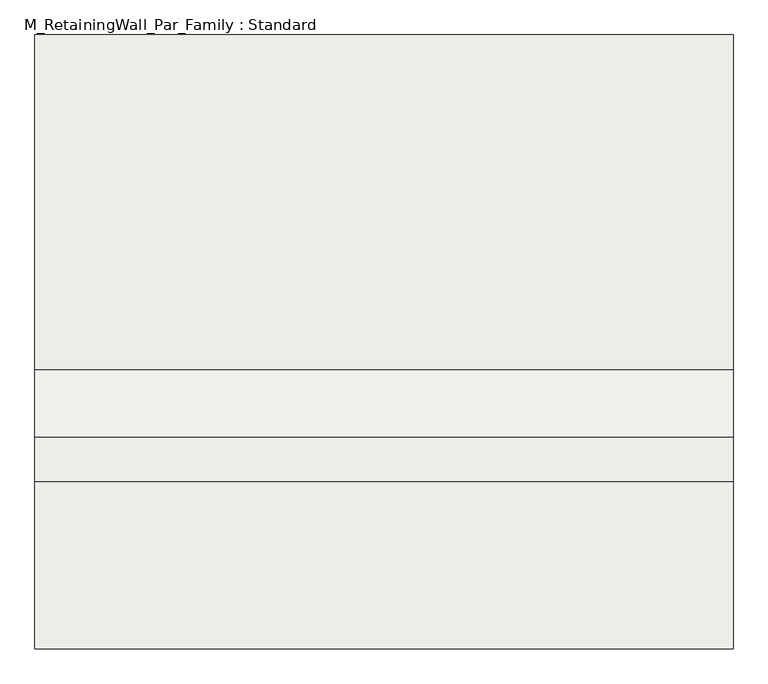
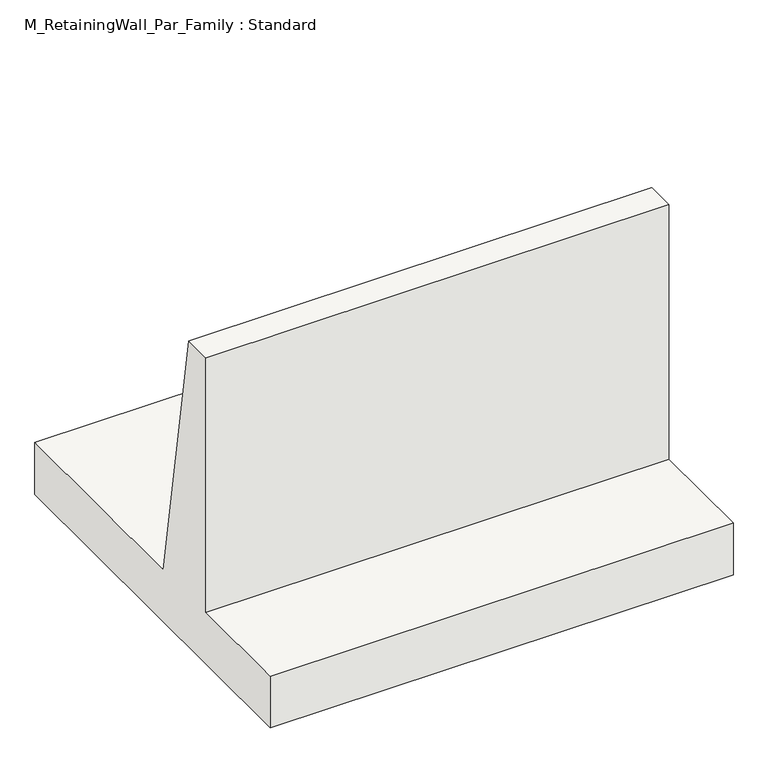
"""IFC4 building model written with IfcOpenShell, lengths in millimetres: slab geometry, M_RetainingWall_Par_Family : Standard."""

from ifc_helpers import new_model, si_unit, frame, origin, place, context, project, spatial, polyline, outline, extrude, source, transform, mapped, element, save


def m_retainingwall_par_family_standard_c8c2fbf1(model_context):
    return source(origin(), model_context, "Body", "SweptSolid", [
        extrude(outline(polyline([(-3200.0, 3500.0), (-2880.4375124, 3500.0), (-2400.0, 592.2), (0.0, 592.2), (0.0, 0.0), (-4400.0, 0.0), (-4400.0, 592.2), (-3200.0, 592.2), (-3200.0, 3500.0)])), frame((0.0, 0.0, 0.0), z_axis=(1.0, 0.0, 0.0), x_axis=(0.0, 1.0, 0.0)), (0.0, 0.0, 1.0), 5000.0),
    ])


if __name__ == "__main__":
    model = new_model("IFC4")
    model_context = context("Model", 3, world=origin())
    ifc_project = project(units=[si_unit("LENGTHUNIT", "METRE", prefix="MILLI")], contexts=[model_context])
    site = spatial("IfcSite", under=ifc_project)
    building = spatial("IfcBuilding", under=site)
    placement = place(None, origin())
    m_retainingwall_par_family_standard_shape = m_retainingwall_par_family_standard_c8c2fbf1(model_context)
    element("IfcSlab", 1, ObjectType="M_RetainingWall_Par_Family : Standard", at=placement, inside=building, context=model_context, shape_type="MappedRepresentation", body=[
        mapped(m_retainingwall_par_family_standard_shape, transform((0.0, 0.0, 0.0), x_axis=(1.0, 0.0, 0.0), y_axis=(0.0, 1.0, 0.0), z_axis=(0.0, 0.0, 1.0))),
    ])
    save(model, "model.ifc")

# Revit data of these elements
# Project information
#   Project Issue Date = "Issue Date"
#   Project Status = "Project Status"
#   Client Name = "Owner"
#   Project Address = "Enter address here"
#   Project Name = "Project Name"
#   Project Number = "0001"
# Type "M_RetainingWall_Par_Family : Standard"
#   hdiff = 61.2 mm
#   h7 = 3026.2 mm
#   h6 = 0 mm
#   h4 = 3026.2 mm
#   h3 = 3087.4 mm
#   Tmp2 = 2271.36 mm
#   Tmp1 = 3200 mm
#   Length [instance default] = 5000 mm
#   H = 3500 mm
#   Gw2 = 800 mm
#   Gw1 = 300 mm
#   Gf4 = 592.2 mm
#   Gamma2 = 9.38186°
#   Gamma = 9.38186°
#   Bw = 2400 mm
#   Beta = 0.00°
#   B = 4400 mm
#   Alpha = 0.00°
#   Structural Material [instance default] = Concrete, Cast-in-Place gray
#   Assembly Code = ""
# Element 1 (IfcSlab, "M_RetainingWall_Par_Family : Standard")
#   Materials on its faces: "Concrete, Cast-in-Place gray"
# Materials
#   "Concrete, Cast-in-Place gray": class "Concrete", colour RGB 192 192 192, transparency 0, Description = "Cast-in-place concrete", Cost = 0
